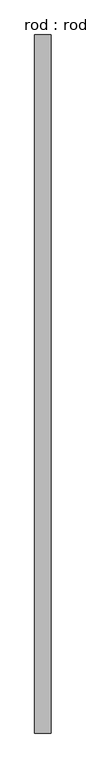
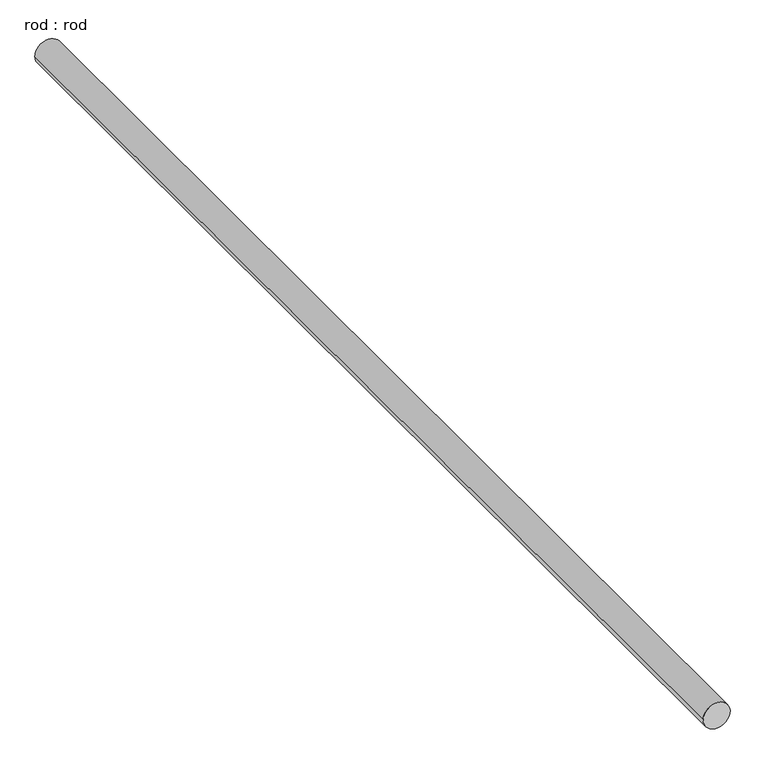
"""IFC4 building model written with IfcOpenShell, lengths in millimetres: proxy geometry, rod : rod."""

from ifc_helpers import new_model, si_unit, point, frame, frame_2d, origin, place, context, project, spatial, circle_curve, trimmed, segment, composite_curve, outline, extrude, source, transform, mapped, element, save


def rod_rod_7b106770(model_context):
    return source(origin(), model_context, "Body", "SweptSolid", [
        extrude(outline(composite_curve([segment(trimmed(circle_curve(frame_2d((0.0108462, 0.0)), 200.0), [point((0.0108462, 200.0))], [point((0.0108462, -200.0))], False, "CARTESIAN"), True, "CONTINUOUS"), segment(trimmed(circle_curve(frame_2d((0.0108462, 0.0)), 200.0), [point((0.0108462, -200.0))], [point((0.0108462, 200.0))], False, "CARTESIAN"), True, "CONTINUOUS")], self_intersect=False)), frame((0.0, -4519.5914118, 0.0), z_axis=(0.0, 1.0, 0.0), x_axis=(0.0, 0.0, 1.0)), (0.0, 0.0, 1.0), 17224.6400543),
    ])


if __name__ == "__main__":
    model = new_model("IFC4")
    model_context = context("Model", 3, world=origin())
    ifc_project = project(units=[si_unit("LENGTHUNIT", "METRE", prefix="MILLI")], contexts=[model_context])
    site = spatial("IfcSite", under=ifc_project)
    building = spatial("IfcBuilding", under=site)
    placement = place(None, origin())
    rod_rod_shape = rod_rod_7b106770(model_context)
    element("IfcBuildingElementProxy", 1, Name="rod : rod", ObjectType="rod : rod", at=placement, inside=building, context=model_context, shape_type="MappedRepresentation", body=[
        mapped(rod_rod_shape, transform((0.0, 0.0, 0.0), x_axis=(1.0, 0.0, 0.0), y_axis=(0.0, 1.0, 0.0), z_axis=(0.0, 0.0, 1.0))),
    ])
    save(model, "model.ifc")

# Revit data of these elements
# Type "rod : rod"
#   Default Elevation = 0
